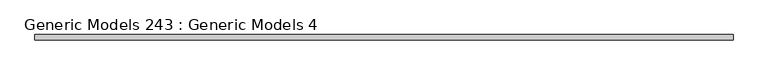
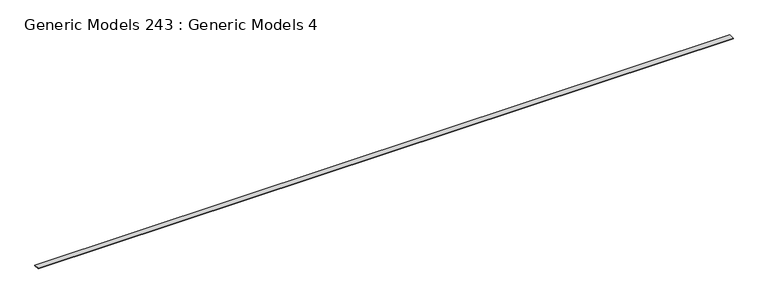
"""IFC4 building model written with IfcOpenShell, lengths in millimetres: proxy geometry, Generic Models 243 : Generic Models 4."""

from ifc_helpers import new_model, si_unit, frame, origin, place, context, project, spatial, polyline, outline, extrude, source, transform, mapped, element, save


def generic_models_243_generic_models_4_8f7382f2(model_context):
    return source(origin(), model_context, "Body", "SweptSolid", [
        extrude(outline(polyline([(13598.6371921, -20170.6690091), (13598.6371921, -20316.38703), (-5044.9628079, -20316.38703), (-5044.9628079, -20170.6690091), (13598.6371921, -20170.6690091)])), frame((0.0, 0.0, 126993.2559733), z_axis=(0.0, 0.0, 1.0), x_axis=(1.0, 0.0, 0.0)), (0.0, 0.0, 1.0), 19.05),
    ])


if __name__ == "__main__":
    model = new_model("IFC4")
    model_context = context("Model", 3, world=origin())
    ifc_project = project(units=[si_unit("LENGTHUNIT", "METRE", prefix="MILLI")], contexts=[model_context])
    site = spatial("IfcSite", under=ifc_project)
    building = spatial("IfcBuilding", under=site)
    placement = place(None, origin())
    generic_models_243_generic_models_4_shape = generic_models_243_generic_models_4_8f7382f2(model_context)
    element("IfcBuildingElementProxy", 1, Name="Generic Models 243 : Generic Models 4", ObjectType="Generic Models 243 : Generic Models 4", at=placement, inside=building, context=model_context, shape_type="MappedRepresentation", body=[
        mapped(generic_models_243_generic_models_4_shape, transform((0.0, 0.0, 0.0), x_axis=(1.0, 0.0, 0.0), y_axis=(0.0, 1.0, 0.0), z_axis=(0.0, 0.0, 1.0))),
    ])
    save(model, "model.ifc")

# Revit data of these elements
# Element 1 (IfcBuildingElementProxy, "Generic Models 243 : Generic Models 4")
#   Materials on its faces: "_CDX PLYWOOD - SEE STRUCT DWGs"
# Materials
#   "_CDX PLYWOOD - SEE STRUCT DWGs": class "Generic", colour RGB 98 75 74, transparency 0, Cost = 0
